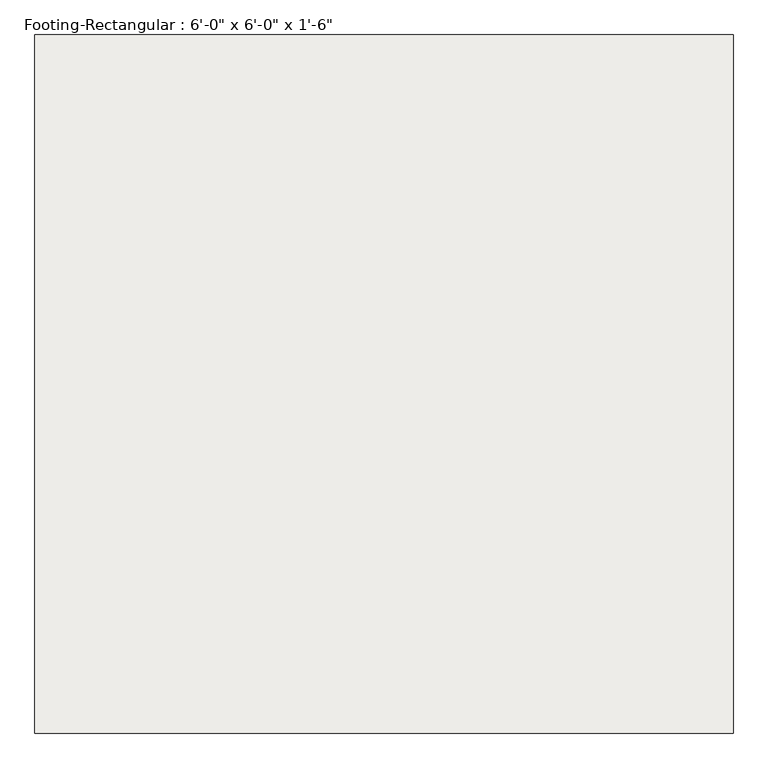
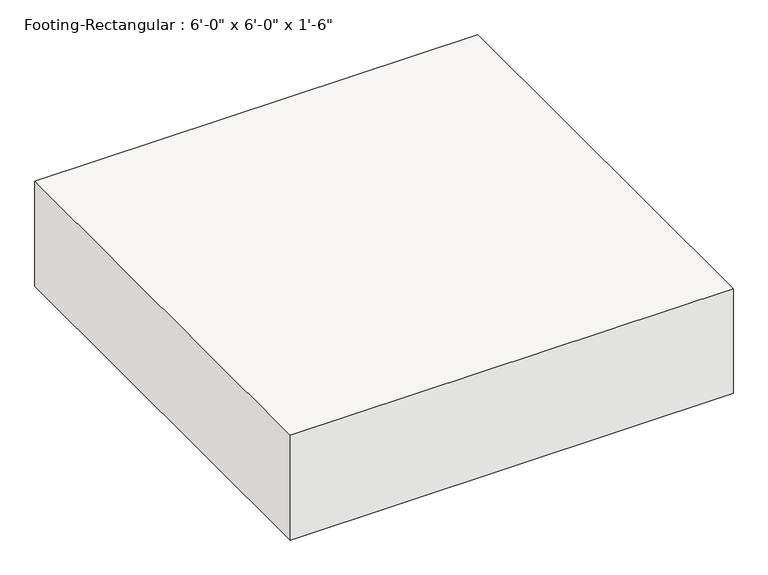
"""IFC4 building model written with IfcOpenShell, lengths in millimetres: slab geometry."""

from ifc_helpers import new_model, si_unit, frame, origin, place, context, project, spatial, polyline, outline, extrude, source, transform, mapped, element, save


def slab_6d6a3403(model_context):
    return source(origin(), model_context, "Body", "SweptSolid", [
        extrude(outline(polyline([(914.4, 914.4), (914.4, -914.4), (-914.4, -914.4), (-914.4, 914.4), (914.4, 914.4)])), frame((0.0, 0.0, -457.2), z_axis=(0.0, 0.0, 1.0), x_axis=(1.0, 0.0, 0.0)), (0.0, 0.0, 1.0), 457.2),
    ])


if __name__ == "__main__":
    model = new_model("IFC4")
    model_context = context("Model", 3, world=origin())
    ifc_project = project(units=[si_unit("LENGTHUNIT", "METRE", prefix="MILLI")], contexts=[model_context])
    site = spatial("IfcSite", under=ifc_project)
    building = spatial("IfcBuilding", under=site)
    placement = place(None, origin())
    slab_shape = slab_6d6a3403(model_context)
    element("IfcSlab", 1, ObjectType="Footing-Rectangular : 6'-0\" x 6'-0\" x 1'-6\"", at=placement, inside=building, context=model_context, shape_type="MappedRepresentation", body=[
        mapped(slab_shape, transform((0.0, 0.0, 0.0), x_axis=(1.0, 0.0, 0.0), y_axis=(0.0, 1.0, 0.0), z_axis=(0.0, 0.0, 1.0))),
    ])
    save(model, "model.ifc")

# Revit data of these elements
# Type "Footing-Rectangular : 6'-0\" x 6'-0\" x 1'-6\""
#   Description = ""
#   Assembly Code = "A1010100"
#   Width = 1828.8 mm
#   Length = 1828.8 mm
#   Thickness = 457.2 mm
#   Structural Material [instance default] = Concrete, Cast-in-Place gray
# Element 1 (IfcSlab, "Footing-Rectangular : 6'-0\" x 6'-0\" x 1'-6\"")
#   Materials on its faces: "Concrete, Cast-in-Place gray"
# Materials
#   "Concrete, Cast-in-Place gray": class "Concrete", colour RGB 192 192 192, transparency 0, Description = "Cast-in-place concrete", Cost = 0
